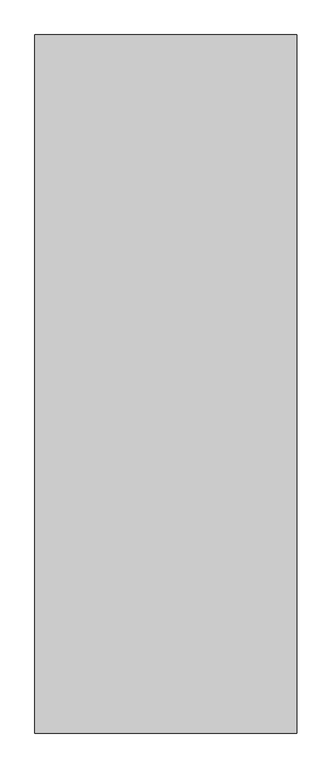
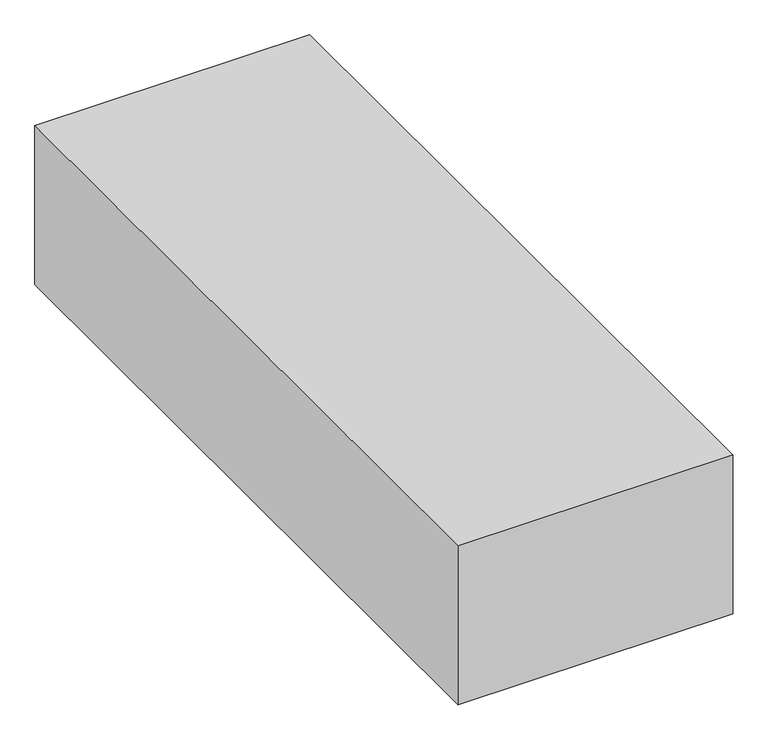
"""IFC4 building model written with IfcOpenShell, lengths in millimetres: proxy geometry, Space Planning Box_hec : Space Planning Box_hec."""

from ifc_helpers import new_model, si_unit, origin, origin_with_axes, place, context, project, spatial, polyline, outline, extrude, source, transform, mapped, element, save


def generic_models_7ea3b148(model_context):
    return source(origin(), model_context, "Body", "SweptSolid", [
        extrude(outline(polyline([(4500.0, 12000.0), (4500.0, -12000.0), (-4500.0, -12000.0), (-4500.0, 12000.0), (4500.0, 12000.0)])), origin_with_axes(), (0.0, 0.0, 1.0), 5500.0),
    ])


if __name__ == "__main__":
    model = new_model("IFC4")
    model_context = context("Model", 3, world=origin())
    ifc_project = project(units=[si_unit("LENGTHUNIT", "METRE", prefix="MILLI")], contexts=[model_context])
    site = spatial("IfcSite", under=ifc_project)
    building = spatial("IfcBuilding", under=site)
    placement = place(None, origin())
    generic_models_shape = generic_models_7ea3b148(model_context)
    element("IfcBuildingElementProxy", 1, Name="Space Planning Box_hec : Space Planning Box_hec", ObjectType="Space Planning Box_hec : Space Planning Box_hec", at=placement, inside=building, context=model_context, shape_type="MappedRepresentation", body=[
        mapped(generic_models_shape, transform((0.0, 0.0, 0.0), x_axis=(1.0, 0.0, 0.0), y_axis=(0.0, 1.0, 0.0), z_axis=(0.0, 0.0, 1.0))),
    ])
    save(model, "model.ifc")

# Revit data of these elements
# Type "Space Planning Box_hec : Space Planning Box_hec"
#   Type Comments = "..."
#   Room Name [instance default] = "?"
#   Interior Finish [instance default] = ""
#   Exterior Finish [instance default] = ""
#   Department [instance default] = ""
#   Assembly Code = "..."
#   ceiling height [instance default] = 0
#   Width [instance default] = 1524 mm
#   Program Area [instance default] = 0.00 m²
#   Length [instance default] = 1524 mm
#   Height [instance default] = 1524 mm
#   Area [instance default] = 2.32258 m²
#   Fill Color [instance default] = Cyan
#   Default Elevation = 0
# Element 1 (IfcBuildingElementProxy, "Space Planning Box_hec : Space Planning Box_hec")
#   Room Name = "Central Control Room"
#   Exterior Finish = "N/A..N/A,,EW1..N/A..N/A"
#   Department = "CI"
#   Width = 9000 mm
#   Program Area = 216.00 m²
#   Length = 24000 mm
#   Height = 5500 mm
#   Area = 216.00 m²
#   Fill Color = Yellow
#   Materials on its faces: "Yellow"
# Materials
#   "Cyan": class "Generic", colour RGB 0 255 255, transparency 0.2, Cost = 0
#   "Yellow": class "Generic", colour RGB 255 255 0, transparency 0.2, Cost = 0
